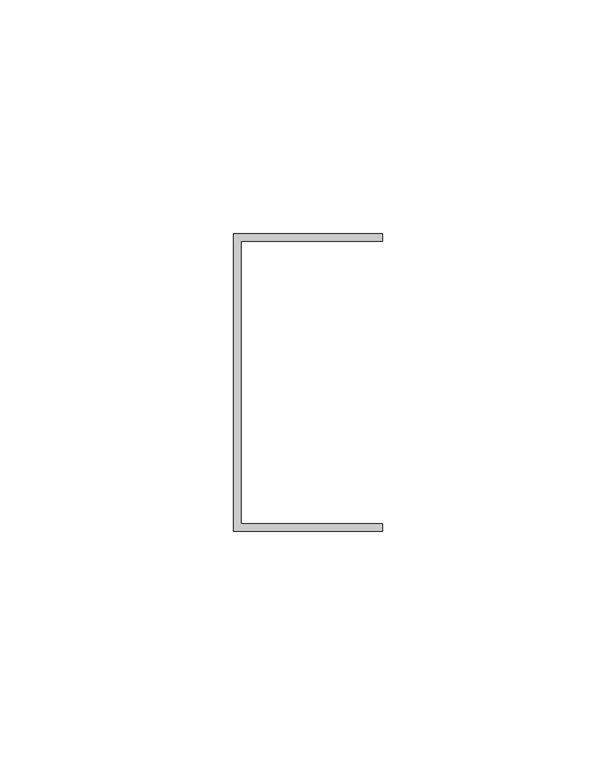
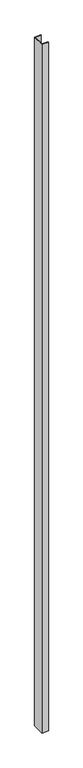
"""IFC4 building model written with IfcOpenShell, lengths in millimetres: proxy geometry, Generic Models 7:Generic Models 1:3:Generic Models 1:3 : Generic Models 7:Generic Models 1:305549:3:Generic Models 1:3:Generic Models 1:3 : Generic Models 7:Generic Models 1:305549:3 : Generic Models 7:Generic Models 1:3:Generic Models 1:3 : Generic Models 7:Generic Models 1:305549:301244:34 : Generic Models 7:Generic Models 1:3:Generic Models 1:3 : Generic Models 7:Generic Models 1:305549:3:Generic Models 1:3:Generic Models 1:3 : Generic Models 7:Generic Models 1:305549:3 : Generic Models 7:Generic Models 1:3:Generic Models 1:3 : Generic Models 7:Generic Models 1:305549:301244:308848."""

from ifc_helpers import new_model, si_unit, frame, origin, place, context, project, spatial, polyline, outline, extrude, source, transform, mapped, element, save


def generic_models_943eb0fb(model_context):
    return source(origin(), model_context, "Body", "SweptSolid", [
        extrude(outline(polyline([(594966.8117239, -579013.3913841), (594998.5617239, -579013.3913841), (594998.5617239, -579014.9788841), (594968.3992239, -579014.9788841), (594968.3992239, -579075.3038841), (594998.5617239, -579075.3038841), (594998.5617239, -579076.8913841), (594966.8117239, -579076.8913841), (594966.8117239, -579013.3913841)])), frame((0.0, 0.0, 38.1), z_axis=(0.0, 0.0, 1.0), x_axis=(1.0, 0.0, 0.0)), (0.0, 0.0, 1.0), 3657.6),
    ])


if __name__ == "__main__":
    model = new_model("IFC4")
    model_context = context("Model", 3, world=origin())
    ifc_project = project(units=[si_unit("LENGTHUNIT", "METRE", prefix="MILLI")], contexts=[model_context])
    site = spatial("IfcSite", under=ifc_project)
    building = spatial("IfcBuilding", under=site)
    placement = place(None, origin())
    generic_models_shape = generic_models_943eb0fb(model_context)
    element("IfcBuildingElementProxy", 1, Name="Generic Models 7:Generic Models 1:3:Generic Models 1:3 : Generic Models 7:Generic Models 1:305549:3:Generic Models 1:3:Generic Models 1:3 : Generic Models 7:Generic Models 1:305549:3 : Generic Models 7:Generic Models 1:3:Generic Models 1:3 : Generic Models 7:Generic Models 1:305549:301244:34 : Generic Models 7:Generic Models 1:3:Generic Models 1:3 : Generic Models 7:Generic Models 1:305549:3:Generic Models 1:3:Generic Models 1:3 : Generic Models 7:Generic Models 1:305549:3 : Generic Models 7:Generic Models 1:3:Generic Models 1:3 : Generic Models 7:Generic Models 1:305549:301244:308848", ObjectType="Generic Models 7:Generic Models 1:3:Generic Models 1:3 : Generic Models 7:Generic Models 1:305549:3:Generic Models 1:3:Generic Models 1:3 : Generic Models 7:Generic Models 1:305549:3 : Generic Models 7:Generic Models 1:3:Generic Models 1:3 : Generic Models 7:Generic Models 1:305549:301244:34 : Generic Models 7:Generic Models 1:3:Generic Models 1:3 : Generic Models 7:Generic Models 1:305549:3:Generic Models 1:3:Generic Models 1:3 : Generic Models 7:Generic Models 1:305549:3 : Generic Models 7:Generic Models 1:3:Generic Models 1:3 : Generic Models 7:Generic Models 1:305549:301244:308848", at=placement, inside=building, context=model_context, shape_type="MappedRepresentation", body=[
        mapped(generic_models_shape, transform((0.0, 0.0, 0.0), x_axis=(1.0, 0.0, 0.0), y_axis=(0.0, 1.0, 0.0), z_axis=(0.0, 0.0, 1.0))),
    ])
    save(model, "model.ifc")

# Revit data of these elements
# Type "Generic Models 7:Generic Models 1:3:Generic Models 1:3 : Generic Models 7:Generic Models 1:305549:3:Generic Models 1:3:Generic Models 1:3 : Generic Models 7:Generic Models 1:305549:3 : Generic Models 7:Generic Models 1:3:Generic Models 1:3 : Generic Models 7:Generic Models 1:305549:301244:34 : Generic Models 7:Generic Models 1:3:Generic Models 1:3 : Generic Models 7:Generic Models 1:305549:3:Generic Models 1:3:Generic Models 1:3 : Generic Models 7:Generic Models 1:305549:3 : Generic Models 7:Generic Models 1:3:Generic Models 1:3 : Generic Models 7:Generic Models 1:305549:301244:308848"
#   NameOverride = "Generic Models 7:Generic Models 1:3:Generic Models 1:3 : Generic Models 7:Generic Models 1:305549:3:Generic Models 1:3:Generic Models 1:3 : Generic Models 7:Generic Models 1:305549:3 : Generic Models 7:Generic Models 1:3:Generic Models 1:3 : Generic Models 7:Generic Models 1:305549:301244:308848"
#   ObjectTypeOverride = "Generic Models 1:3:Generic Models 1:3 : Generic Models 7:Generic Models 1:305549:3 : Generic Models 7:Generic Models 1:3:Generic Models 1:3 : Generic Models 7:Generic Models 1:305549:301244"
#   Reference = "Generic Models 1"
#   Tag = "308848"
# Element 1 (IfcBuildingElementProxy, "Generic Models 7:Generic Models 1:3:Generic Models 1:3 : Generic Models 7:Generic Models 1:305549:3:Generic Models 1:3:Generic Models 1:3 : Generic Models 7:Generic Models 1:305549:3 : Generic Models 7:Generic Models 1:3:Generic Models 1:3 : Generic Models 7:Generic Models 1:305549:301244:34 : Generic Models 7:Generic Models 1:3:Generic Models 1:3 : Generic Models 7:Generic Models 1:305549:3:Generic Models 1:3:Generic Models 1:3 : Generic Models 7:Generic Models 1:305549:3 : Generic Models 7:Generic Models 1:3:Generic Models 1:3 : Generic Models 7:Generic Models 1:305549:301244:308848")
#   Materials on its faces: "GALVANIZED U-CHANNEL (250T125-33)"
# Materials
#   "GALVANIZED U-CHANNEL (250T125-33)": class "Unassigned", colour RGB 202 201 200, transparency 0, Keynote = "M05451300.02", Cost = 0
